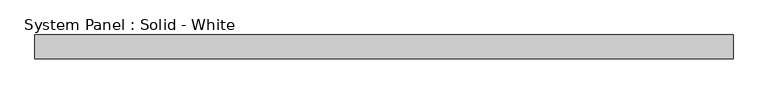
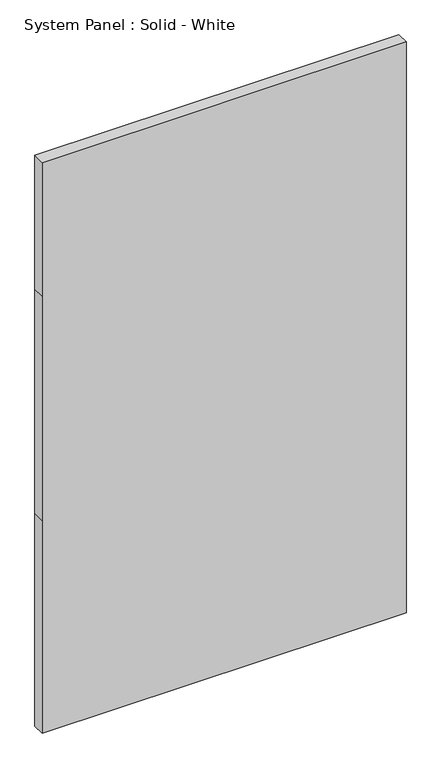
"""IFC4 building model written with IfcOpenShell, lengths in millimetres: plate geometry, System Panel : Solid - White."""

from ifc_helpers import new_model, si_unit, frame, origin, place, context, project, spatial, polyline, outline, extrude, source, transform, mapped, element, save


def system_panel_solid_white_ad8f58d9(model_context):
    return source(origin(), model_context, "Body", "SweptSolid", [
        extrude(outline(polyline([(0.0, -936.0121469), (0.0, 936.0121469), (1155.7, 936.0121469), (2374.9, 936.0121469), (3101.9419949, 936.0121469), (3101.9419949, -936.0121469), (2374.9, -936.0121469), (1155.7, -936.0121469), (0.0, -936.0121469)])), frame((0.0, -44.45, 0.0), z_axis=(0.0, 1.0, 0.0), x_axis=(0.0, 0.0, 1.0)), (0.0, 0.0, 1.0), 63.5),
    ])


if __name__ == "__main__":
    model = new_model("IFC4")
    model_context = context("Model", 3, world=origin())
    ifc_project = project(units=[si_unit("LENGTHUNIT", "METRE", prefix="MILLI")], contexts=[model_context])
    site = spatial("IfcSite", under=ifc_project)
    building = spatial("IfcBuilding", under=site)
    placement = place(None, origin())
    system_panel_solid_white_shape = system_panel_solid_white_ad8f58d9(model_context)
    element("IfcPlate", 1, ObjectType="System Panel : Solid - White", at=placement, inside=building, context=model_context, shape_type="MappedRepresentation", body=[
        mapped(system_panel_solid_white_shape, transform((0.0, 0.0, 0.0), x_axis=(1.0, 0.0, 0.0), y_axis=(0.0, 1.0, 0.0), z_axis=(0.0, 0.0, 1.0))),
    ])
    save(model, "model.ifc")

# Revit data of these elements
# Element 1 (IfcPlate, "System Panel : Solid - White")
#   Materials on its faces: "White Panel"
# Materials
#   "White Panel": class "Unassigned", colour RGB 255 255 255, transparency 0
